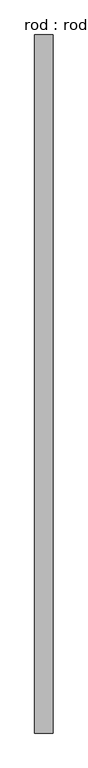
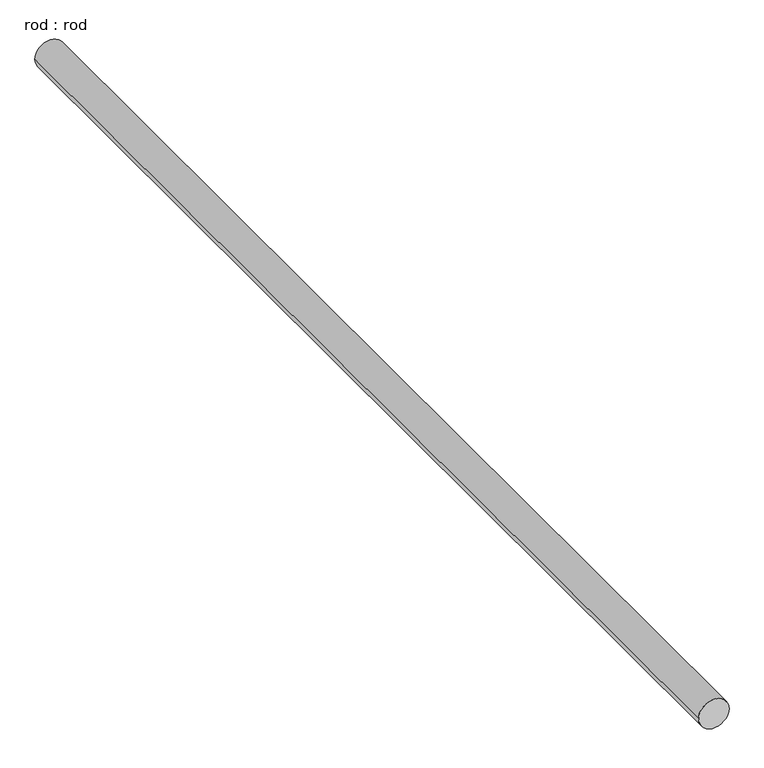
"""IFC4 building model written with IfcOpenShell, lengths in millimetres: proxy geometry, rod : rod."""

import ifcopenshell
import ifcopenshell.guid

model = None  # the IFC model being written
_history = None  # IfcOwnerHistory: only IFC2X3 demands one
_inside = {}  # id of a spatial element -> (the spatial element, [elements in it])
_under = {}  # id of a project, library or spatial element -> (it, [spatial elements below it])
_declared = {}  # id of a project -> (the project, [libraries it declares])
_typed = {}  # id of a type object -> (the type object, [elements of that type])
_made_of = {}  # id of a material, layer set ... -> (it, [elements and type objects made of it])


def new_model(schema):
    """Start an empty IFC model of exactly this schema.

    Asked for "IFC4X3", IfcOpenShell would pick the latest addendum, in which some entities
    have other attributes; the version numbers below select the first issue.
    IFC2X3 requires an IfcOwnerHistory on every rooted entity: one is made here for all.
    """
    global model, _history
    if schema == "IFC4X3":
        model = ifcopenshell.file(schema_version=(4, 3, 0, 0))
    else:
        model = ifcopenshell.file(schema=schema)
    _inside.clear()
    _under.clear()
    _declared.clear()
    _typed.clear()
    _made_of.clear()
    _history = None
    if model.schema == "IFC2X3":
        org = make("IfcOrganization", Name="unknown")
        user = make(
            "IfcPersonAndOrganization",
            ThePerson=make("IfcPerson", FamilyName="unknown"),
            TheOrganization=org,
        )
        app = make(
            "IfcApplication",
            ApplicationDeveloper=org,
            Version="unknown",
            ApplicationFullName="unknown",
            ApplicationIdentifier="unknown",
        )
        _history = make(
            "IfcOwnerHistory",
            OwningUser=user,
            OwningApplication=app,
            ChangeAction="ADDED",
            CreationDate=0,
        )
    return model


def make(cls, **values):
    """One entity of the class cls with the attributes given. An attribute that is None is left unset."""
    return model.create_entity(
        cls, **{name: value for name, value in values.items() if value is not None}
    )


def rooted(cls, **values):
    """An entity with a GlobalId (a new one), such as an element, a storey or a relation."""
    return make(cls, GlobalId=ifcopenshell.guid.new(), OwnerHistory=_history, **values)


def si_unit(unit_type, name, prefix=None):
    """IfcSIUnit, for example si_unit("LENGTHUNIT", "METRE", prefix="MILLI")."""
    return make("IfcSIUnit", UnitType=unit_type, Prefix=prefix, Name=name)


def assignment(units):
    """IfcUnitAssignment: the units of a project."""
    return None if units is None else make("IfcUnitAssignment", Units=units)


def point(xyz):
    """IfcCartesianPoint."""
    return None if xyz is None else make("IfcCartesianPoint", Coordinates=xyz)


def direction(xyz):
    """IfcDirection."""
    return None if xyz is None else make("IfcDirection", DirectionRatios=xyz)


def frame(location, z_axis=None, x_axis=None):
    """IfcAxis2Placement3D, a coordinate frame: its origin and axes. An axis left out is left unset."""
    return make(
        "IfcAxis2Placement3D",
        Location=point(location),
        Axis=direction(z_axis),
        RefDirection=direction(x_axis),
    )


def frame_2d(location, x_axis=None):
    """IfcAxis2Placement2D, a coordinate frame in the plane: its origin and x axis."""
    return make(
        "IfcAxis2Placement2D", Location=point(location), RefDirection=direction(x_axis)
    )


def origin():
    """The frame at (0, 0, 0) with its axes left unset."""
    return frame((0.0, 0.0, 0.0))


def place(relative_to, where):
    """IfcLocalPlacement: puts the frame where relative to a parent placement (None: the world)."""
    return make(
        "IfcLocalPlacement", PlacementRelTo=relative_to, RelativePlacement=where
    )


def context(
    kind, dimensions, precision=None, world=None, true_north=None, identifier=None
):
    """IfcGeometricRepresentationContext, for example the 3D "Model" context."""
    return make(
        "IfcGeometricRepresentationContext",
        ContextIdentifier=identifier,
        ContextType=kind,
        CoordinateSpaceDimension=dimensions,
        Precision=precision,
        WorldCoordinateSystem=world,
        TrueNorth=true_north,
    )


def project(units=None, contexts=None):
    """IfcProject with its units and contexts."""
    return rooted(
        "IfcProject",
        Name="project",
        RepresentationContexts=contexts,
        UnitsInContext=assignment(units),
    )


def spatial(cls, under=None, at=None, **own):
    """A site, building, storey or space (cls), placed at a placement, below another one or the project."""
    s = rooted(cls, ObjectPlacement=at, **own)
    if under is not None:
        _under.setdefault(under.id(), (under, []))[1].append(s)
    return s


def circle_curve(where, radius):
    """IfcCircle in the frame where."""
    return make("IfcCircle", Position=where, Radius=radius)


def trimmed(basis, trim1, trim2, sense, master):
    """IfcTrimmedCurve: the piece of a basis curve between two trims."""
    return make(
        "IfcTrimmedCurve",
        BasisCurve=basis,
        Trim1=trim1,
        Trim2=trim2,
        SenseAgreement=sense,
        MasterRepresentation=master,
    )


def segment(curve, same_sense, transition):
    """IfcCompositeCurveSegment."""
    return make(
        "IfcCompositeCurveSegment",
        Transition=transition,
        SameSense=same_sense,
        ParentCurve=curve,
    )


def composite_curve(segments, self_intersect=None):
    """IfcCompositeCurve: segments joined end to end."""
    return make("IfcCompositeCurve", Segments=segments, SelfIntersect=self_intersect)


def outline(outer, holes=None, kind="AREA"):
    """IfcArbitraryClosedProfileDef: a profile drawn as a closed curve; with holes, ...WithVoids."""
    if holes is None:
        return make("IfcArbitraryClosedProfileDef", ProfileType=kind, OuterCurve=outer)
    return make(
        "IfcArbitraryProfileDefWithVoids",
        ProfileType=kind,
        OuterCurve=outer,
        InnerCurves=holes,
    )


def extrude(swept, where, along, depth):
    """IfcExtrudedAreaSolid: the profile swept, set in the frame where, extruded along a direction by depth."""
    return make(
        "IfcExtrudedAreaSolid",
        SweptArea=swept,
        Position=where,
        ExtrudedDirection=direction(along),
        Depth=depth,
    )


def shape(context_of_items, identifier, shape_type, items):
    """IfcShapeRepresentation: the items that make up one representation, for example the "Body"."""
    return make(
        "IfcShapeRepresentation",
        ContextOfItems=context_of_items,
        RepresentationIdentifier=identifier,
        RepresentationType=shape_type,
        Items=items,
    )


def source(mapping_origin, context_of_items, identifier, shape_type, items):
    """IfcRepresentationMap: a shape defined once, which mapped items show again and again."""
    return make(
        "IfcRepresentationMap",
        MappingOrigin=mapping_origin,
        MappedRepresentation=shape(context_of_items, identifier, shape_type, items),
    )


def transform(
    local_origin,
    x_axis=None,
    y_axis=None,
    z_axis=None,
    scale=None,
    scale2=None,
    scale3=None,
    uniform=True,
):
    """IfcCartesianTransformationOperator3D, or its non-uniform kind. x_axis, y_axis, z_axis: its Axis1, 2, 3."""
    if uniform:
        return make(
            "IfcCartesianTransformationOperator3D",
            Axis1=direction(x_axis),
            Axis2=direction(y_axis),
            LocalOrigin=point(local_origin),
            Scale=scale,
            Axis3=direction(z_axis),
        )
    return make(
        "IfcCartesianTransformationOperator3DnonUniform",
        Axis1=direction(x_axis),
        Axis2=direction(y_axis),
        LocalOrigin=point(local_origin),
        Scale=scale,
        Axis3=direction(z_axis),
        Scale2=scale2,
        Scale3=scale3,
    )


def mapped(mapping_source, mapping_target):
    """IfcMappedItem: shows the shape of a source again, moved by a transform."""
    return make(
        "IfcMappedItem", MappingSource=mapping_source, MappingTarget=mapping_target
    )


def made_of(thing, what):
    """Note that an element or type object is made of a material, layer set ...; save() writes the relation."""
    if what is not None:
        _made_of.setdefault(what.id(), (what, []))[1].append(thing)
    return thing


def element(
    cls,
    number,
    at=None,
    inside=None,
    cuts=None,
    type_object=None,
    material=None,
    context=None,
    identifier="Body",
    shape_type=None,
    held_by="IfcProductDefinitionShape",
    body=None,
    shapes=None,
    **own,
):
    """One element of the class cls, such as IfcWall. Its Tag is "e" and its number.

    at: its placement. inside: the storey or other place that contains it. cuts: it is an
    opening in that element (IfcRelVoidsElement). A single representation is given by context,
    identifier, shape_type and body (its items); several are given by shapes. held_by: the class
    of the entity that holds the representations. save() writes the other relations.
    """
    e = rooted(cls, Tag="e%d" % number, ObjectPlacement=at, **own)
    if body is not None:
        shapes = [shape(context, identifier, shape_type, body)]
    if shapes is not None:
        e.Representation = make(held_by, Representations=shapes)
    if inside is not None:
        _inside.setdefault(inside.id(), (inside, []))[1].append(e)
    if cuts is not None:
        rooted(
            "IfcRelVoidsElement", RelatingBuildingElement=cuts, RelatedOpeningElement=e
        )
    if type_object is not None:
        _typed.setdefault(type_object.id(), (type_object, []))[1].append(e)
    return made_of(e, material)


def aggregate(whole, parts):
    """IfcRelAggregates: a whole, such as a stair, and the parts it consists of."""
    return rooted("IfcRelAggregates", RelatingObject=whole, RelatedObjects=parts)


def save(model, path):
    """Write the relations noted so far, then the file.

    IfcRelAggregates (storeys below a building ...), IfcRelContainedInSpatialStructure (elements
    in a storey), IfcRelDefinesByType, IfcRelAssociatesMaterial and IfcRelDeclares: one each for
    every whole, place, type object, material and project.
    """
    for whole, parts in _under.values():
        aggregate(whole, parts)
    for where, things in _inside.values():
        rooted(
            "IfcRelContainedInSpatialStructure",
            RelatedElements=things,
            RelatingStructure=where,
        )
    for kind, things in _typed.values():
        rooted("IfcRelDefinesByType", RelatedObjects=things, RelatingType=kind)
    for what, things in _made_of.values():
        rooted("IfcRelAssociatesMaterial", RelatedObjects=things, RelatingMaterial=what)
    for by, libraries in _declared.values():
        rooted("IfcRelDeclares", RelatingContext=by, RelatedDefinitions=libraries)
    model.write(path)


def rod_rod_29761a59(model_context):
    return source(origin(), model_context, "Body", "SweptSolid", [
        extrude(outline(composite_curve([segment(trimmed(circle_curve(frame_2d((0.0108462, 0.0)), 200.0), [point((0.0108462, 200.0))], [point((0.0108462, -200.0))], False, "CARTESIAN"), True, "CONTINUOUS"), segment(trimmed(circle_curve(frame_2d((0.0108462, 0.0)), 200.0), [point((0.0108462, -200.0))], [point((0.0108462, 200.0))], False, "CARTESIAN"), True, "CONTINUOUS")], self_intersect=False)), frame((0.0, -3471.3806156, 0.0), z_axis=(0.0, 1.0, 0.0), x_axis=(0.0, 0.0, 1.0)), (0.0, 0.0, 1.0), 15128.2184618),
    ])


if __name__ == "__main__":
    model = new_model("IFC4")
    model_context = context("Model", 3, world=origin())
    ifc_project = project(units=[si_unit("LENGTHUNIT", "METRE", prefix="MILLI")], contexts=[model_context])
    site = spatial("IfcSite", under=ifc_project)
    building = spatial("IfcBuilding", under=site)
    placement = place(None, origin())
    rod_rod_shape = rod_rod_29761a59(model_context)
    element("IfcBuildingElementProxy", 1, Name="rod : rod", ObjectType="rod : rod", at=placement, inside=building, context=model_context, shape_type="MappedRepresentation", body=[
        mapped(rod_rod_shape, transform((0.0, 0.0, 0.0), x_axis=(1.0, 0.0, 0.0), y_axis=(0.0, 1.0, 0.0), z_axis=(0.0, 0.0, 1.0))),
    ])
    save(model, "model.ifc")

# Revit data of these elements
# Type "rod : rod"
#   Default Elevation = 0
